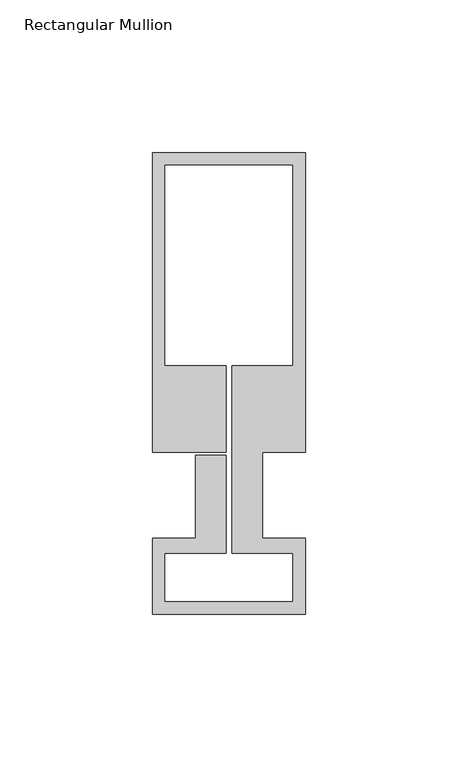
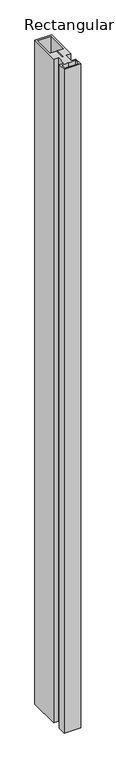
"""IFC4 building model written with IfcOpenShell, lengths in millimetres: member geometry, Rectangular Mullion : Schueco_FWS-50-HI_Mull_CovCap-20mm_Mull-85mm."""

from ifc_helpers import new_model, si_unit, frame, origin, place, context, project, spatial, polyline, outline, extrude, source, transform, mapped, element, save


def rectangular_mullion_35cf74e1(model_context):
    return source(origin(), model_context, "Body", "SweptSolid", [
        extrude(outline(polyline([(0.0, 126.0), (0.0, 28.0), (-14.0, 28.0), (-14.0, -0.1), (0.0, -0.1), (0.0, -25.0), (-50.0, -25.0), (-50.0, -0.1), (-36.0, -0.1), (-36.0, 27.0), (-26.0, 27.0), (-26.0, -5.0), (-46.0, -5.0), (-46.0, -21.0), (-4.0, -21.0), (-4.0, -5.0), (-24.0, -5.0), (-24.0, 56.3), (-4.0, 56.3), (-4.0, 122.0), (-46.0, 122.0), (-46.0, 56.3), (-26.0, 56.3), (-26.0, 28.0), (-50.0, 28.0), (-50.0, 126.0), (0.0, 126.0)])), frame((0.0, 0.0, -2100.0), z_axis=(0.0, 0.0, 1.0), x_axis=(1.0, 0.0, 0.0)), (0.0, 0.0, 1.0), 2100.0),
    ])


if __name__ == "__main__":
    model = new_model("IFC4")
    model_context = context("Model", 3, world=origin())
    ifc_project = project(units=[si_unit("LENGTHUNIT", "METRE", prefix="MILLI")], contexts=[model_context])
    site = spatial("IfcSite", under=ifc_project)
    building = spatial("IfcBuilding", under=site)
    placement = place(None, origin())
    rectangular_mullion_shape = rectangular_mullion_35cf74e1(model_context)
    element("IfcMember", 1, ObjectType="Rectangular Mullion : Schueco_FWS-50-HI_Mull_CovCap-20mm_Mull-85mm", at=placement, inside=building, context=model_context, shape_type="MappedRepresentation", body=[
        mapped(rectangular_mullion_shape, transform((0.0, 0.0, 0.0), x_axis=(1.0, 0.0, 0.0), y_axis=(0.0, 1.0, 0.0), z_axis=(0.0, 0.0, 1.0))),
    ])
    save(model, "model.ifc")

# Revit data of these elements
# Type "Rectangular Mullion : Schueco_FWS-50-HI_Mull_CovCap-20mm_Mull-85mm"
#   Model = "FWS 50.HI"
#   Manufacturer = "Schueco International KG"
#   Type Comments = "Mullion"
#   Schueco thermal insulation standard = "Highly thermally insulated"
#   Burglar resistance = "RC 3"
#   Thermal insulation = "to 0.90 W/(m²K)"
#   built-in parameter 1007322 = 0.495407 (stored number, unit not read)
#   built-in parameter 1007321 = 0.0360892 (stored number, unit not read)
#   built-in parameter 1007320 = 0.0360892 (stored number, unit not read)
# Element 1 (IfcMember, "Rectangular Mullion : Schueco_FWS-50-HI_Mull_CovCap-20mm_Mull-85mm")
#   Materials on its faces: "Alu"
# Materials
#   "Alu": class "Glas", colour RGB 140 140 140, transparency 0
